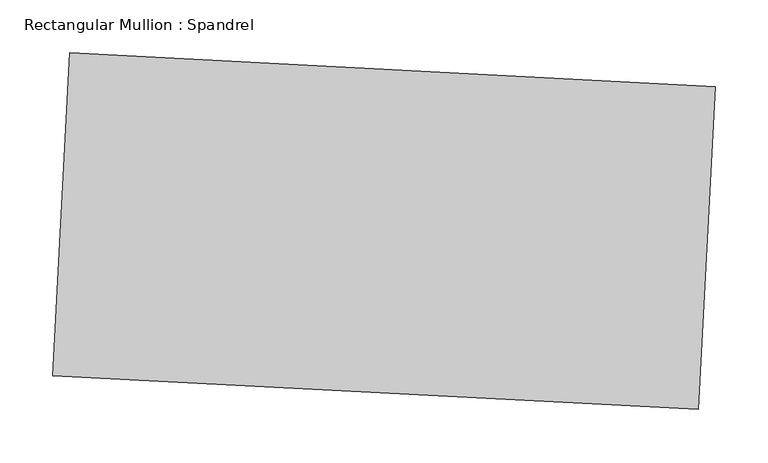
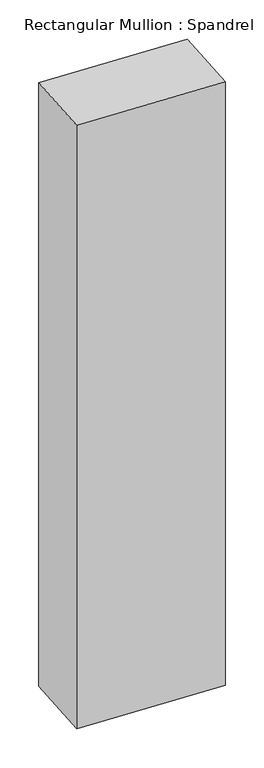
"""IFC4 building model written with IfcOpenShell, lengths in millimetres: member geometry, Rectangular Mullion : Spandrel."""

import ifcopenshell
import ifcopenshell.guid

model = None  # the IFC model being written
_history = None  # IfcOwnerHistory: only IFC2X3 demands one
_inside = {}  # id of a spatial element -> (the spatial element, [elements in it])
_under = {}  # id of a project, library or spatial element -> (it, [spatial elements below it])
_declared = {}  # id of a project -> (the project, [libraries it declares])
_typed = {}  # id of a type object -> (the type object, [elements of that type])
_made_of = {}  # id of a material, layer set ... -> (it, [elements and type objects made of it])


def new_model(schema):
    """Start an empty IFC model of exactly this schema.

    Asked for "IFC4X3", IfcOpenShell would pick the latest addendum, in which some entities
    have other attributes; the version numbers below select the first issue.
    IFC2X3 requires an IfcOwnerHistory on every rooted entity: one is made here for all.
    """
    global model, _history
    if schema == "IFC4X3":
        model = ifcopenshell.file(schema_version=(4, 3, 0, 0))
    else:
        model = ifcopenshell.file(schema=schema)
    _inside.clear()
    _under.clear()
    _declared.clear()
    _typed.clear()
    _made_of.clear()
    _history = None
    if model.schema == "IFC2X3":
        org = make("IfcOrganization", Name="unknown")
        user = make(
            "IfcPersonAndOrganization",
            ThePerson=make("IfcPerson", FamilyName="unknown"),
            TheOrganization=org,
        )
        app = make(
            "IfcApplication",
            ApplicationDeveloper=org,
            Version="unknown",
            ApplicationFullName="unknown",
            ApplicationIdentifier="unknown",
        )
        _history = make(
            "IfcOwnerHistory",
            OwningUser=user,
            OwningApplication=app,
            ChangeAction="ADDED",
            CreationDate=0,
        )
    return model


def make(cls, **values):
    """One entity of the class cls with the attributes given. An attribute that is None is left unset."""
    return model.create_entity(
        cls, **{name: value for name, value in values.items() if value is not None}
    )


def rooted(cls, **values):
    """An entity with a GlobalId (a new one), such as an element, a storey or a relation."""
    return make(cls, GlobalId=ifcopenshell.guid.new(), OwnerHistory=_history, **values)


def si_unit(unit_type, name, prefix=None):
    """IfcSIUnit, for example si_unit("LENGTHUNIT", "METRE", prefix="MILLI")."""
    return make("IfcSIUnit", UnitType=unit_type, Prefix=prefix, Name=name)


def assignment(units):
    """IfcUnitAssignment: the units of a project."""
    return None if units is None else make("IfcUnitAssignment", Units=units)


def point(xyz):
    """IfcCartesianPoint."""
    return None if xyz is None else make("IfcCartesianPoint", Coordinates=xyz)


def direction(xyz):
    """IfcDirection."""
    return None if xyz is None else make("IfcDirection", DirectionRatios=xyz)


def frame(location, z_axis=None, x_axis=None):
    """IfcAxis2Placement3D, a coordinate frame: its origin and axes. An axis left out is left unset."""
    return make(
        "IfcAxis2Placement3D",
        Location=point(location),
        Axis=direction(z_axis),
        RefDirection=direction(x_axis),
    )


def origin():
    """The frame at (0, 0, 0) with its axes left unset."""
    return frame((0.0, 0.0, 0.0))


def place(relative_to, where):
    """IfcLocalPlacement: puts the frame where relative to a parent placement (None: the world)."""
    return make(
        "IfcLocalPlacement", PlacementRelTo=relative_to, RelativePlacement=where
    )


def context(
    kind, dimensions, precision=None, world=None, true_north=None, identifier=None
):
    """IfcGeometricRepresentationContext, for example the 3D "Model" context."""
    return make(
        "IfcGeometricRepresentationContext",
        ContextIdentifier=identifier,
        ContextType=kind,
        CoordinateSpaceDimension=dimensions,
        Precision=precision,
        WorldCoordinateSystem=world,
        TrueNorth=true_north,
    )


def project(units=None, contexts=None):
    """IfcProject with its units and contexts."""
    return rooted(
        "IfcProject",
        Name="project",
        RepresentationContexts=contexts,
        UnitsInContext=assignment(units),
    )


def spatial(cls, under=None, at=None, **own):
    """A site, building, storey or space (cls), placed at a placement, below another one or the project."""
    s = rooted(cls, ObjectPlacement=at, **own)
    if under is not None:
        _under.setdefault(under.id(), (under, []))[1].append(s)
    return s


def polyline(points):
    """IfcPolyline through the points."""
    return make("IfcPolyline", Points=[point(p) for p in points])


def outline(outer, holes=None, kind="AREA"):
    """IfcArbitraryClosedProfileDef: a profile drawn as a closed curve; with holes, ...WithVoids."""
    if holes is None:
        return make("IfcArbitraryClosedProfileDef", ProfileType=kind, OuterCurve=outer)
    return make(
        "IfcArbitraryProfileDefWithVoids",
        ProfileType=kind,
        OuterCurve=outer,
        InnerCurves=holes,
    )


def extrude(swept, where, along, depth):
    """IfcExtrudedAreaSolid: the profile swept, set in the frame where, extruded along a direction by depth."""
    return make(
        "IfcExtrudedAreaSolid",
        SweptArea=swept,
        Position=where,
        ExtrudedDirection=direction(along),
        Depth=depth,
    )


def shape(context_of_items, identifier, shape_type, items):
    """IfcShapeRepresentation: the items that make up one representation, for example the "Body"."""
    return make(
        "IfcShapeRepresentation",
        ContextOfItems=context_of_items,
        RepresentationIdentifier=identifier,
        RepresentationType=shape_type,
        Items=items,
    )


def source(mapping_origin, context_of_items, identifier, shape_type, items):
    """IfcRepresentationMap: a shape defined once, which mapped items show again and again."""
    return make(
        "IfcRepresentationMap",
        MappingOrigin=mapping_origin,
        MappedRepresentation=shape(context_of_items, identifier, shape_type, items),
    )


def transform(
    local_origin,
    x_axis=None,
    y_axis=None,
    z_axis=None,
    scale=None,
    scale2=None,
    scale3=None,
    uniform=True,
):
    """IfcCartesianTransformationOperator3D, or its non-uniform kind. x_axis, y_axis, z_axis: its Axis1, 2, 3."""
    if uniform:
        return make(
            "IfcCartesianTransformationOperator3D",
            Axis1=direction(x_axis),
            Axis2=direction(y_axis),
            LocalOrigin=point(local_origin),
            Scale=scale,
            Axis3=direction(z_axis),
        )
    return make(
        "IfcCartesianTransformationOperator3DnonUniform",
        Axis1=direction(x_axis),
        Axis2=direction(y_axis),
        LocalOrigin=point(local_origin),
        Scale=scale,
        Axis3=direction(z_axis),
        Scale2=scale2,
        Scale3=scale3,
    )


def mapped(mapping_source, mapping_target):
    """IfcMappedItem: shows the shape of a source again, moved by a transform."""
    return make(
        "IfcMappedItem", MappingSource=mapping_source, MappingTarget=mapping_target
    )


def made_of(thing, what):
    """Note that an element or type object is made of a material, layer set ...; save() writes the relation."""
    if what is not None:
        _made_of.setdefault(what.id(), (what, []))[1].append(thing)
    return thing


def element(
    cls,
    number,
    at=None,
    inside=None,
    cuts=None,
    type_object=None,
    material=None,
    context=None,
    identifier="Body",
    shape_type=None,
    held_by="IfcProductDefinitionShape",
    body=None,
    shapes=None,
    **own,
):
    """One element of the class cls, such as IfcWall. Its Tag is "e" and its number.

    at: its placement. inside: the storey or other place that contains it. cuts: it is an
    opening in that element (IfcRelVoidsElement). A single representation is given by context,
    identifier, shape_type and body (its items); several are given by shapes. held_by: the class
    of the entity that holds the representations. save() writes the other relations.
    """
    e = rooted(cls, Tag="e%d" % number, ObjectPlacement=at, **own)
    if body is not None:
        shapes = [shape(context, identifier, shape_type, body)]
    if shapes is not None:
        e.Representation = make(held_by, Representations=shapes)
    if inside is not None:
        _inside.setdefault(inside.id(), (inside, []))[1].append(e)
    if cuts is not None:
        rooted(
            "IfcRelVoidsElement", RelatingBuildingElement=cuts, RelatedOpeningElement=e
        )
    if type_object is not None:
        _typed.setdefault(type_object.id(), (type_object, []))[1].append(e)
    return made_of(e, material)


def aggregate(whole, parts):
    """IfcRelAggregates: a whole, such as a stair, and the parts it consists of."""
    return rooted("IfcRelAggregates", RelatingObject=whole, RelatedObjects=parts)


def save(model, path):
    """Write the relations noted so far, then the file.

    IfcRelAggregates (storeys below a building ...), IfcRelContainedInSpatialStructure (elements
    in a storey), IfcRelDefinesByType, IfcRelAssociatesMaterial and IfcRelDeclares: one each for
    every whole, place, type object, material and project.
    """
    for whole, parts in _under.values():
        aggregate(whole, parts)
    for where, things in _inside.values():
        rooted(
            "IfcRelContainedInSpatialStructure",
            RelatedElements=things,
            RelatingStructure=where,
        )
    for kind, things in _typed.values():
        rooted("IfcRelDefinesByType", RelatedObjects=things, RelatingType=kind)
    for what, things in _made_of.values():
        rooted("IfcRelAssociatesMaterial", RelatedObjects=things, RelatingMaterial=what)
    for by, libraries in _declared.values():
        rooted("IfcRelDeclares", RelatingContext=by, RelatedDefinitions=libraries)
    model.write(path)


def rectangular_mullion_spandrel_57f4b63b(model_context):
    return source(origin(), model_context, "Body", "SweptSolid", [
        extrude(outline(polyline([(312.3582819, 136.2391416), (296.4062825, -168.1431406), (-312.3582819, -136.2391416), (-296.4062825, 168.1431406), (312.3582819, 136.2391416)])), frame((0.0, 0.0, -2693.0670444), z_axis=(0.0, 0.0, 1.0), x_axis=(1.0, 0.0, 0.0)), (0.0, 0.0, 1.0), 2693.0670444),
    ])


if __name__ == "__main__":
    model = new_model("IFC4")
    model_context = context("Model", 3, world=origin())
    ifc_project = project(units=[si_unit("LENGTHUNIT", "METRE", prefix="MILLI")], contexts=[model_context])
    site = spatial("IfcSite", under=ifc_project)
    building = spatial("IfcBuilding", under=site)
    placement = place(None, origin())
    rectangular_mullion_spandrel_shape = rectangular_mullion_spandrel_57f4b63b(model_context)
    element("IfcMember", 1, ObjectType="Rectangular Mullion : Spandrel", at=placement, inside=building, context=model_context, shape_type="MappedRepresentation", body=[
        mapped(rectangular_mullion_spandrel_shape, transform((0.0, 0.0, 0.0), x_axis=(1.0, 0.0, 0.0), y_axis=(0.0, 1.0, 0.0), z_axis=(0.0, 0.0, 1.0))),
    ])
    save(model, "model.ifc")

# Revit data of these elements
# Type "Rectangular Mullion : Spandrel"
#   built-in parameter 1007304 = 1 (stored number, unit not read)
#   built-in parameter 1007301 = 1 (stored number, unit not read)
#   built-in parameter 1007300 = 1 (stored number, unit not read)
# Element 1 (IfcMember, "Rectangular Mullion : Spandrel")
#   Materials on its faces: "Aluminum"
# Materials
#   "Aluminum": class "Metal", colour RGB 247 247 247, transparency 0, Description = "Aluminum 6061", Cost = 0
